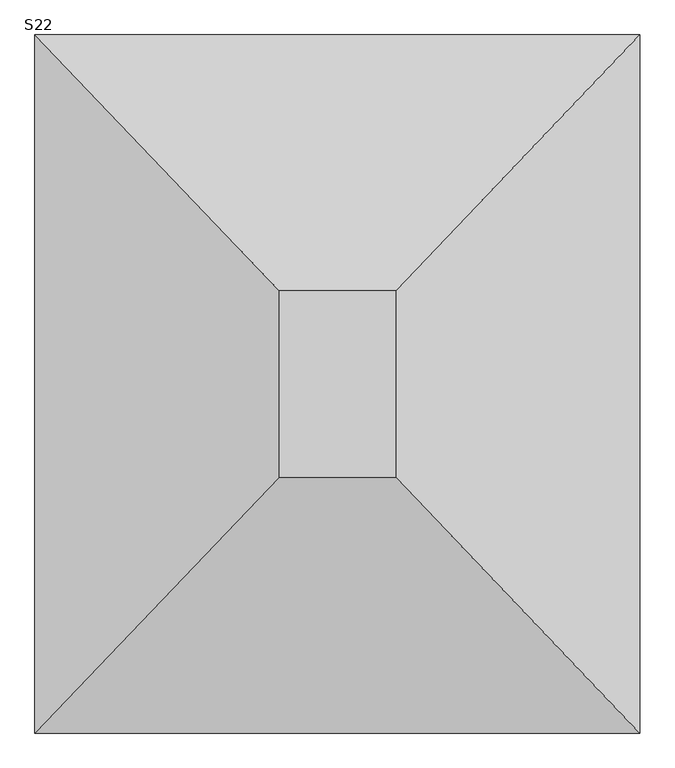
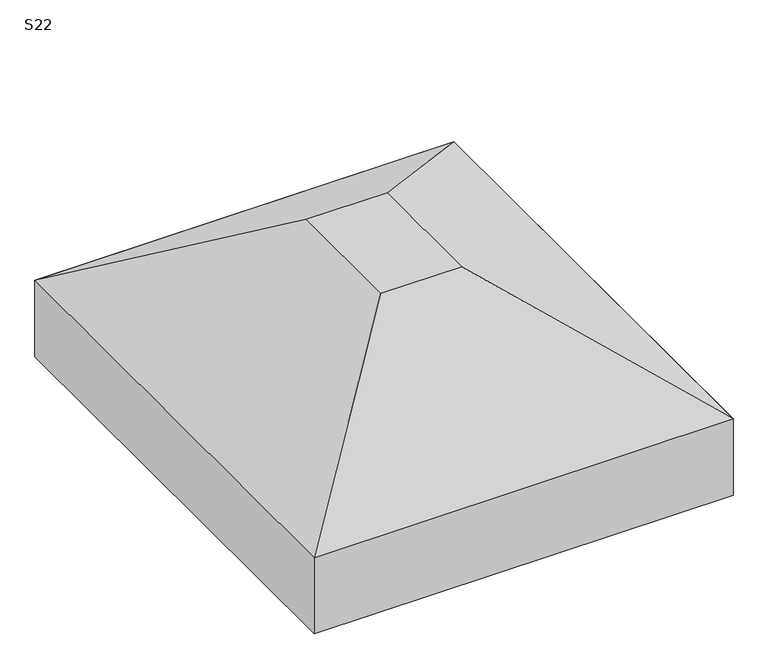
"""IFC4 building model written with IfcOpenShell, lengths in millimetres: fastener geometry, TQS - Sapata : S22."""

import ifcopenshell
import ifcopenshell.guid

model = None  # the IFC model being written
_history = None  # IfcOwnerHistory: only IFC2X3 demands one
_inside = {}  # id of a spatial element -> (the spatial element, [elements in it])
_under = {}  # id of a project, library or spatial element -> (it, [spatial elements below it])
_declared = {}  # id of a project -> (the project, [libraries it declares])
_typed = {}  # id of a type object -> (the type object, [elements of that type])
_made_of = {}  # id of a material, layer set ... -> (it, [elements and type objects made of it])


def new_model(schema):
    """Start an empty IFC model of exactly this schema.

    Asked for "IFC4X3", IfcOpenShell would pick the latest addendum, in which some entities
    have other attributes; the version numbers below select the first issue.
    IFC2X3 requires an IfcOwnerHistory on every rooted entity: one is made here for all.
    """
    global model, _history
    if schema == "IFC4X3":
        model = ifcopenshell.file(schema_version=(4, 3, 0, 0))
    else:
        model = ifcopenshell.file(schema=schema)
    _inside.clear()
    _under.clear()
    _declared.clear()
    _typed.clear()
    _made_of.clear()
    _history = None
    if model.schema == "IFC2X3":
        org = make("IfcOrganization", Name="unknown")
        user = make(
            "IfcPersonAndOrganization",
            ThePerson=make("IfcPerson", FamilyName="unknown"),
            TheOrganization=org,
        )
        app = make(
            "IfcApplication",
            ApplicationDeveloper=org,
            Version="unknown",
            ApplicationFullName="unknown",
            ApplicationIdentifier="unknown",
        )
        _history = make(
            "IfcOwnerHistory",
            OwningUser=user,
            OwningApplication=app,
            ChangeAction="ADDED",
            CreationDate=0,
        )
    return model


def make(cls, **values):
    """One entity of the class cls with the attributes given. An attribute that is None is left unset."""
    return model.create_entity(
        cls, **{name: value for name, value in values.items() if value is not None}
    )


def rooted(cls, **values):
    """An entity with a GlobalId (a new one), such as an element, a storey or a relation."""
    return make(cls, GlobalId=ifcopenshell.guid.new(), OwnerHistory=_history, **values)


def si_unit(unit_type, name, prefix=None):
    """IfcSIUnit, for example si_unit("LENGTHUNIT", "METRE", prefix="MILLI")."""
    return make("IfcSIUnit", UnitType=unit_type, Prefix=prefix, Name=name)


def assignment(units):
    """IfcUnitAssignment: the units of a project."""
    return None if units is None else make("IfcUnitAssignment", Units=units)


def point(xyz):
    """IfcCartesianPoint."""
    return None if xyz is None else make("IfcCartesianPoint", Coordinates=xyz)


def direction(xyz):
    """IfcDirection."""
    return None if xyz is None else make("IfcDirection", DirectionRatios=xyz)


def frame(location, z_axis=None, x_axis=None):
    """IfcAxis2Placement3D, a coordinate frame: its origin and axes. An axis left out is left unset."""
    return make(
        "IfcAxis2Placement3D",
        Location=point(location),
        Axis=direction(z_axis),
        RefDirection=direction(x_axis),
    )


def origin():
    """The frame at (0, 0, 0) with its axes left unset."""
    return frame((0.0, 0.0, 0.0))


def place(relative_to, where):
    """IfcLocalPlacement: puts the frame where relative to a parent placement (None: the world)."""
    return make(
        "IfcLocalPlacement", PlacementRelTo=relative_to, RelativePlacement=where
    )


def context(
    kind, dimensions, precision=None, world=None, true_north=None, identifier=None
):
    """IfcGeometricRepresentationContext, for example the 3D "Model" context."""
    return make(
        "IfcGeometricRepresentationContext",
        ContextIdentifier=identifier,
        ContextType=kind,
        CoordinateSpaceDimension=dimensions,
        Precision=precision,
        WorldCoordinateSystem=world,
        TrueNorth=true_north,
    )


def project(units=None, contexts=None):
    """IfcProject with its units and contexts."""
    return rooted(
        "IfcProject",
        Name="project",
        RepresentationContexts=contexts,
        UnitsInContext=assignment(units),
    )


def spatial(cls, under=None, at=None, **own):
    """A site, building, storey or space (cls), placed at a placement, below another one or the project."""
    s = rooted(cls, ObjectPlacement=at, **own)
    if under is not None:
        _under.setdefault(under.id(), (under, []))[1].append(s)
    return s


def polyline(points):
    """IfcPolyline through the points."""
    return make("IfcPolyline", Points=[point(p) for p in points])


def outline(outer, holes=None, kind="AREA"):
    """IfcArbitraryClosedProfileDef: a profile drawn as a closed curve; with holes, ...WithVoids."""
    if holes is None:
        return make("IfcArbitraryClosedProfileDef", ProfileType=kind, OuterCurve=outer)
    return make(
        "IfcArbitraryProfileDefWithVoids",
        ProfileType=kind,
        OuterCurve=outer,
        InnerCurves=holes,
    )


def extrude(swept, where, along, depth):
    """IfcExtrudedAreaSolid: the profile swept, set in the frame where, extruded along a direction by depth."""
    return make(
        "IfcExtrudedAreaSolid",
        SweptArea=swept,
        Position=where,
        ExtrudedDirection=direction(along),
        Depth=depth,
    )


def faces_of(points, faces, orient=None, outer=None):
    """IfcFace entities. A face is a list of loops; a loop is a list of indices into points, from 0.

    orient and outer hold one flag for each loop. By default every Orientation is true, the
    first loop of a face is its IfcFaceOuterBound and the others are IfcFaceBound.
    """
    made = []
    for i, loops in enumerate(faces):
        bounds = []
        for j, loop in enumerate(loops):
            is_outer = j == 0 if outer is None else outer[i][j]
            bounds.append(
                make(
                    "IfcFaceOuterBound" if is_outer else "IfcFaceBound",
                    Bound=make("IfcPolyLoop", Polygon=[points[k] for k in loop]),
                    Orientation=True if orient is None else orient[i][j],
                )
            )
        made.append(make("IfcFace", Bounds=bounds))
    return made


def faceted_brep(points, faces, orient=None, outer=None, voids=None):
    """IfcFacetedBrep: a solid bounded by flat faces; with voids (closed shells), ...WithVoids."""
    shared = [point(p) for p in points]
    hull = make("IfcClosedShell", CfsFaces=faces_of(shared, faces, orient, outer))
    if voids is None:
        return make("IfcFacetedBrep", Outer=hull)
    return make(
        "IfcFacetedBrepWithVoids",
        Outer=hull,
        Voids=[
            make(cls, CfsFaces=faces_of(shared, fs, o, b)) for cls, fs, o, b in voids
        ],
    )


def shape(context_of_items, identifier, shape_type, items):
    """IfcShapeRepresentation: the items that make up one representation, for example the "Body"."""
    return make(
        "IfcShapeRepresentation",
        ContextOfItems=context_of_items,
        RepresentationIdentifier=identifier,
        RepresentationType=shape_type,
        Items=items,
    )


def source(mapping_origin, context_of_items, identifier, shape_type, items):
    """IfcRepresentationMap: a shape defined once, which mapped items show again and again."""
    return make(
        "IfcRepresentationMap",
        MappingOrigin=mapping_origin,
        MappedRepresentation=shape(context_of_items, identifier, shape_type, items),
    )


def transform(
    local_origin,
    x_axis=None,
    y_axis=None,
    z_axis=None,
    scale=None,
    scale2=None,
    scale3=None,
    uniform=True,
):
    """IfcCartesianTransformationOperator3D, or its non-uniform kind. x_axis, y_axis, z_axis: its Axis1, 2, 3."""
    if uniform:
        return make(
            "IfcCartesianTransformationOperator3D",
            Axis1=direction(x_axis),
            Axis2=direction(y_axis),
            LocalOrigin=point(local_origin),
            Scale=scale,
            Axis3=direction(z_axis),
        )
    return make(
        "IfcCartesianTransformationOperator3DnonUniform",
        Axis1=direction(x_axis),
        Axis2=direction(y_axis),
        LocalOrigin=point(local_origin),
        Scale=scale,
        Axis3=direction(z_axis),
        Scale2=scale2,
        Scale3=scale3,
    )


def mapped(mapping_source, mapping_target):
    """IfcMappedItem: shows the shape of a source again, moved by a transform."""
    return make(
        "IfcMappedItem", MappingSource=mapping_source, MappingTarget=mapping_target
    )


def made_of(thing, what):
    """Note that an element or type object is made of a material, layer set ...; save() writes the relation."""
    if what is not None:
        _made_of.setdefault(what.id(), (what, []))[1].append(thing)
    return thing


def element(
    cls,
    number,
    at=None,
    inside=None,
    cuts=None,
    type_object=None,
    material=None,
    context=None,
    identifier="Body",
    shape_type=None,
    held_by="IfcProductDefinitionShape",
    body=None,
    shapes=None,
    **own,
):
    """One element of the class cls, such as IfcWall. Its Tag is "e" and its number.

    at: its placement. inside: the storey or other place that contains it. cuts: it is an
    opening in that element (IfcRelVoidsElement). A single representation is given by context,
    identifier, shape_type and body (its items); several are given by shapes. held_by: the class
    of the entity that holds the representations. save() writes the other relations.
    """
    e = rooted(cls, Tag="e%d" % number, ObjectPlacement=at, **own)
    if body is not None:
        shapes = [shape(context, identifier, shape_type, body)]
    if shapes is not None:
        e.Representation = make(held_by, Representations=shapes)
    if inside is not None:
        _inside.setdefault(inside.id(), (inside, []))[1].append(e)
    if cuts is not None:
        rooted(
            "IfcRelVoidsElement", RelatingBuildingElement=cuts, RelatedOpeningElement=e
        )
    if type_object is not None:
        _typed.setdefault(type_object.id(), (type_object, []))[1].append(e)
    return made_of(e, material)


def aggregate(whole, parts):
    """IfcRelAggregates: a whole, such as a stair, and the parts it consists of."""
    return rooted("IfcRelAggregates", RelatingObject=whole, RelatedObjects=parts)


def save(model, path):
    """Write the relations noted so far, then the file.

    IfcRelAggregates (storeys below a building ...), IfcRelContainedInSpatialStructure (elements
    in a storey), IfcRelDefinesByType, IfcRelAssociatesMaterial and IfcRelDeclares: one each for
    every whole, place, type object, material and project.
    """
    for whole, parts in _under.values():
        aggregate(whole, parts)
    for where, things in _inside.values():
        rooted(
            "IfcRelContainedInSpatialStructure",
            RelatedElements=things,
            RelatingStructure=where,
        )
    for kind, things in _typed.values():
        rooted("IfcRelDefinesByType", RelatedObjects=things, RelatingType=kind)
    for what, things in _made_of.values():
        rooted("IfcRelAssociatesMaterial", RelatedObjects=things, RelatingMaterial=what)
    for by, libraries in _declared.values():
        rooted("IfcRelDeclares", RelatingContext=by, RelatedDefinitions=libraries)
    model.write(path)


def s22_9d23c3d3(model_context):
    return source(origin(), model_context, "Body", "SolidModel", [
        faceted_brep([(-75.0, 0.0, 0.0), (-325.0, 0.0, 0.0), (-325.0, -400.0, 0.0), (-75.0, -400.0, 0.0), (450.0, 550.0, -350.0), (450.0, -950.0, -350.0), (-850.0, -950.0, -350.0), (-850.0, 550.0, -350.0)], [[[0, 1, 2, 3]], [[4, 5, 6, 7]], [[4, 7, 1, 0]], [[7, 6, 2, 1]], [[6, 5, 3, 2]], [[5, 4, 0, 3]]]),
        extrude(outline(polyline([(450.0, 550.0), (450.0, -950.0), (-850.0, -950.0), (-850.0, 550.0), (450.0, 550.0)])), frame((0.0, 0.0, -600.0), z_axis=(0.0, 0.0, 1.0), x_axis=(1.0, 0.0, 0.0)), (0.0, 0.0, 1.0), 250.0),
    ])


if __name__ == "__main__":
    model = new_model("IFC4")
    model_context = context("Model", 3, world=origin())
    ifc_project = project(units=[si_unit("LENGTHUNIT", "METRE", prefix="MILLI")], contexts=[model_context])
    site = spatial("IfcSite", under=ifc_project)
    building = spatial("IfcBuilding", under=site)
    placement = place(None, origin())
    s22_shape = s22_9d23c3d3(model_context)
    element("IfcFastener", 1, ObjectType="TQS - Sapata : S22", at=placement, inside=building, context=model_context, shape_type="MappedRepresentation", body=[
        mapped(s22_shape, transform((0.0, 0.0, 0.0), x_axis=(1.0, 0.0, 0.0), y_axis=(0.0, 1.0, 0.0), z_axis=(0.0, 0.0, 1.0))),
    ])
    save(model, "model.ifc")

# Revit data of these elements
# Type "TQS - Sapata : S22"
#   TY = 0.40 m
#   TX = 0.25 m
#   HS = 0.60 m
#   H0 = 0.25 m
#   EXCYABS = 0.75 m
#   EXCY = 0.00 m
#   EXCXABS = 0.65 m
#   EXCX = 0.00 m
#   DIMY = 1.50 m
#   DIMX = 1.30 m
#   Material estrutural = Concreto - Concreto concretado no local
#   Width = 0
#   Length = 0
# Element 1 (IfcFastener, "TQS - Sapata : S22")
#   Materials on its faces: "Concreto - Concreto concretado no local"
# Materials
#   "Concreto - Concreto concretado no local": class "Concreto", colour RGB 192 192 192, transparency 0
